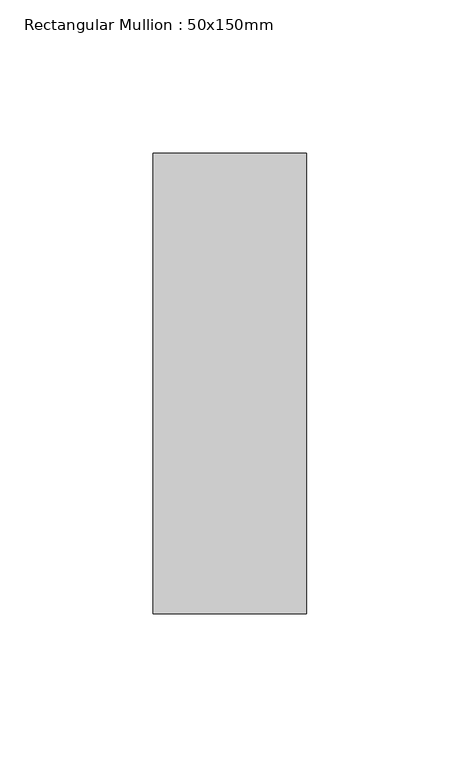
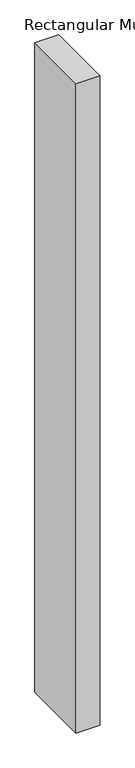
"""IFC4 building model written with IfcOpenShell, lengths in millimetres: member geometry, Rectangular Mullion : 50x150mm."""

import ifcopenshell
import ifcopenshell.guid

model = None  # the IFC model being written
_history = None  # IfcOwnerHistory: only IFC2X3 demands one
_inside = {}  # id of a spatial element -> (the spatial element, [elements in it])
_under = {}  # id of a project, library or spatial element -> (it, [spatial elements below it])
_declared = {}  # id of a project -> (the project, [libraries it declares])
_typed = {}  # id of a type object -> (the type object, [elements of that type])
_made_of = {}  # id of a material, layer set ... -> (it, [elements and type objects made of it])


def new_model(schema):
    """Start an empty IFC model of exactly this schema.

    Asked for "IFC4X3", IfcOpenShell would pick the latest addendum, in which some entities
    have other attributes; the version numbers below select the first issue.
    IFC2X3 requires an IfcOwnerHistory on every rooted entity: one is made here for all.
    """
    global model, _history
    if schema == "IFC4X3":
        model = ifcopenshell.file(schema_version=(4, 3, 0, 0))
    else:
        model = ifcopenshell.file(schema=schema)
    _inside.clear()
    _under.clear()
    _declared.clear()
    _typed.clear()
    _made_of.clear()
    _history = None
    if model.schema == "IFC2X3":
        org = make("IfcOrganization", Name="unknown")
        user = make(
            "IfcPersonAndOrganization",
            ThePerson=make("IfcPerson", FamilyName="unknown"),
            TheOrganization=org,
        )
        app = make(
            "IfcApplication",
            ApplicationDeveloper=org,
            Version="unknown",
            ApplicationFullName="unknown",
            ApplicationIdentifier="unknown",
        )
        _history = make(
            "IfcOwnerHistory",
            OwningUser=user,
            OwningApplication=app,
            ChangeAction="ADDED",
            CreationDate=0,
        )
    return model


def make(cls, **values):
    """One entity of the class cls with the attributes given. An attribute that is None is left unset."""
    return model.create_entity(
        cls, **{name: value for name, value in values.items() if value is not None}
    )


def rooted(cls, **values):
    """An entity with a GlobalId (a new one), such as an element, a storey or a relation."""
    return make(cls, GlobalId=ifcopenshell.guid.new(), OwnerHistory=_history, **values)


def si_unit(unit_type, name, prefix=None):
    """IfcSIUnit, for example si_unit("LENGTHUNIT", "METRE", prefix="MILLI")."""
    return make("IfcSIUnit", UnitType=unit_type, Prefix=prefix, Name=name)


def assignment(units):
    """IfcUnitAssignment: the units of a project."""
    return None if units is None else make("IfcUnitAssignment", Units=units)


def point(xyz):
    """IfcCartesianPoint."""
    return None if xyz is None else make("IfcCartesianPoint", Coordinates=xyz)


def direction(xyz):
    """IfcDirection."""
    return None if xyz is None else make("IfcDirection", DirectionRatios=xyz)


def frame(location, z_axis=None, x_axis=None):
    """IfcAxis2Placement3D, a coordinate frame: its origin and axes. An axis left out is left unset."""
    return make(
        "IfcAxis2Placement3D",
        Location=point(location),
        Axis=direction(z_axis),
        RefDirection=direction(x_axis),
    )


def origin():
    """The frame at (0, 0, 0) with its axes left unset."""
    return frame((0.0, 0.0, 0.0))


def place(relative_to, where):
    """IfcLocalPlacement: puts the frame where relative to a parent placement (None: the world)."""
    return make(
        "IfcLocalPlacement", PlacementRelTo=relative_to, RelativePlacement=where
    )


def context(
    kind, dimensions, precision=None, world=None, true_north=None, identifier=None
):
    """IfcGeometricRepresentationContext, for example the 3D "Model" context."""
    return make(
        "IfcGeometricRepresentationContext",
        ContextIdentifier=identifier,
        ContextType=kind,
        CoordinateSpaceDimension=dimensions,
        Precision=precision,
        WorldCoordinateSystem=world,
        TrueNorth=true_north,
    )


def project(units=None, contexts=None):
    """IfcProject with its units and contexts."""
    return rooted(
        "IfcProject",
        Name="project",
        RepresentationContexts=contexts,
        UnitsInContext=assignment(units),
    )


def spatial(cls, under=None, at=None, **own):
    """A site, building, storey or space (cls), placed at a placement, below another one or the project."""
    s = rooted(cls, ObjectPlacement=at, **own)
    if under is not None:
        _under.setdefault(under.id(), (under, []))[1].append(s)
    return s


def polyline(points):
    """IfcPolyline through the points."""
    return make("IfcPolyline", Points=[point(p) for p in points])


def outline(outer, holes=None, kind="AREA"):
    """IfcArbitraryClosedProfileDef: a profile drawn as a closed curve; with holes, ...WithVoids."""
    if holes is None:
        return make("IfcArbitraryClosedProfileDef", ProfileType=kind, OuterCurve=outer)
    return make(
        "IfcArbitraryProfileDefWithVoids",
        ProfileType=kind,
        OuterCurve=outer,
        InnerCurves=holes,
    )


def extrude(swept, where, along, depth):
    """IfcExtrudedAreaSolid: the profile swept, set in the frame where, extruded along a direction by depth."""
    return make(
        "IfcExtrudedAreaSolid",
        SweptArea=swept,
        Position=where,
        ExtrudedDirection=direction(along),
        Depth=depth,
    )


def shape(context_of_items, identifier, shape_type, items):
    """IfcShapeRepresentation: the items that make up one representation, for example the "Body"."""
    return make(
        "IfcShapeRepresentation",
        ContextOfItems=context_of_items,
        RepresentationIdentifier=identifier,
        RepresentationType=shape_type,
        Items=items,
    )


def source(mapping_origin, context_of_items, identifier, shape_type, items):
    """IfcRepresentationMap: a shape defined once, which mapped items show again and again."""
    return make(
        "IfcRepresentationMap",
        MappingOrigin=mapping_origin,
        MappedRepresentation=shape(context_of_items, identifier, shape_type, items),
    )


def transform(
    local_origin,
    x_axis=None,
    y_axis=None,
    z_axis=None,
    scale=None,
    scale2=None,
    scale3=None,
    uniform=True,
):
    """IfcCartesianTransformationOperator3D, or its non-uniform kind. x_axis, y_axis, z_axis: its Axis1, 2, 3."""
    if uniform:
        return make(
            "IfcCartesianTransformationOperator3D",
            Axis1=direction(x_axis),
            Axis2=direction(y_axis),
            LocalOrigin=point(local_origin),
            Scale=scale,
            Axis3=direction(z_axis),
        )
    return make(
        "IfcCartesianTransformationOperator3DnonUniform",
        Axis1=direction(x_axis),
        Axis2=direction(y_axis),
        LocalOrigin=point(local_origin),
        Scale=scale,
        Axis3=direction(z_axis),
        Scale2=scale2,
        Scale3=scale3,
    )


def mapped(mapping_source, mapping_target):
    """IfcMappedItem: shows the shape of a source again, moved by a transform."""
    return make(
        "IfcMappedItem", MappingSource=mapping_source, MappingTarget=mapping_target
    )


def made_of(thing, what):
    """Note that an element or type object is made of a material, layer set ...; save() writes the relation."""
    if what is not None:
        _made_of.setdefault(what.id(), (what, []))[1].append(thing)
    return thing


def element(
    cls,
    number,
    at=None,
    inside=None,
    cuts=None,
    type_object=None,
    material=None,
    context=None,
    identifier="Body",
    shape_type=None,
    held_by="IfcProductDefinitionShape",
    body=None,
    shapes=None,
    **own,
):
    """One element of the class cls, such as IfcWall. Its Tag is "e" and its number.

    at: its placement. inside: the storey or other place that contains it. cuts: it is an
    opening in that element (IfcRelVoidsElement). A single representation is given by context,
    identifier, shape_type and body (its items); several are given by shapes. held_by: the class
    of the entity that holds the representations. save() writes the other relations.
    """
    e = rooted(cls, Tag="e%d" % number, ObjectPlacement=at, **own)
    if body is not None:
        shapes = [shape(context, identifier, shape_type, body)]
    if shapes is not None:
        e.Representation = make(held_by, Representations=shapes)
    if inside is not None:
        _inside.setdefault(inside.id(), (inside, []))[1].append(e)
    if cuts is not None:
        rooted(
            "IfcRelVoidsElement", RelatingBuildingElement=cuts, RelatedOpeningElement=e
        )
    if type_object is not None:
        _typed.setdefault(type_object.id(), (type_object, []))[1].append(e)
    return made_of(e, material)


def aggregate(whole, parts):
    """IfcRelAggregates: a whole, such as a stair, and the parts it consists of."""
    return rooted("IfcRelAggregates", RelatingObject=whole, RelatedObjects=parts)


def save(model, path):
    """Write the relations noted so far, then the file.

    IfcRelAggregates (storeys below a building ...), IfcRelContainedInSpatialStructure (elements
    in a storey), IfcRelDefinesByType, IfcRelAssociatesMaterial and IfcRelDeclares: one each for
    every whole, place, type object, material and project.
    """
    for whole, parts in _under.values():
        aggregate(whole, parts)
    for where, things in _inside.values():
        rooted(
            "IfcRelContainedInSpatialStructure",
            RelatedElements=things,
            RelatingStructure=where,
        )
    for kind, things in _typed.values():
        rooted("IfcRelDefinesByType", RelatedObjects=things, RelatingType=kind)
    for what, things in _made_of.values():
        rooted("IfcRelAssociatesMaterial", RelatedObjects=things, RelatingMaterial=what)
    for by, libraries in _declared.values():
        rooted("IfcRelDeclares", RelatingContext=by, RelatedDefinitions=libraries)
    model.write(path)


def rectangular_mullion_50x150mm_e3a7335b(model_context):
    return source(origin(), model_context, "Body", "SweptSolid", [
        extrude(outline(polyline([(0.0, 75.0), (0.0, -75.0), (-50.0, -75.0), (-50.0, 75.0), (0.0, 75.0)])), frame((0.0, 0.0, -1449.9999998), z_axis=(0.0, 0.0, 1.0), x_axis=(1.0, 0.0, 0.0)), (0.0, 0.0, 1.0), 1449.9999998),
    ])


if __name__ == "__main__":
    model = new_model("IFC4")
    model_context = context("Model", 3, world=origin())
    ifc_project = project(units=[si_unit("LENGTHUNIT", "METRE", prefix="MILLI")], contexts=[model_context])
    site = spatial("IfcSite", under=ifc_project)
    building = spatial("IfcBuilding", under=site)
    placement = place(None, origin())
    rectangular_mullion_50x150mm_shape = rectangular_mullion_50x150mm_e3a7335b(model_context)
    element("IfcMember", 1, ObjectType="Rectangular Mullion : 50x150mm", at=placement, inside=building, context=model_context, shape_type="MappedRepresentation", body=[
        mapped(rectangular_mullion_50x150mm_shape, transform((0.0, 0.0, 0.0), x_axis=(1.0, 0.0, 0.0), y_axis=(0.0, 1.0, 0.0), z_axis=(0.0, 0.0, 1.0))),
    ])
    save(model, "model.ifc")

# Revit data of these elements
# Type "Rectangular Mullion : 50x150mm"
#   Keynote = "H11"
#   built-in parameter 1007304 = 0.492126 (stored number, unit not read)
#   built-in parameter 1007301 = 0.082021 (stored number, unit not read)
#   built-in parameter 1007300 = 0.082021 (stored number, unit not read)
# Element 1 (IfcMember, "Rectangular Mullion : 50x150mm")
#   Materials on its faces: "Aluminium"
# Materials
#   "Aluminium": class "Metal", colour RGB 247 247 247, transparency 0, Description = "Aluminium 6061", Cost = 0
